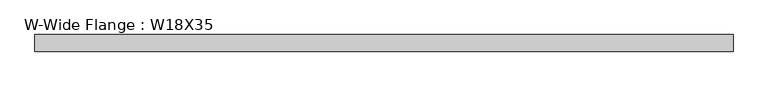
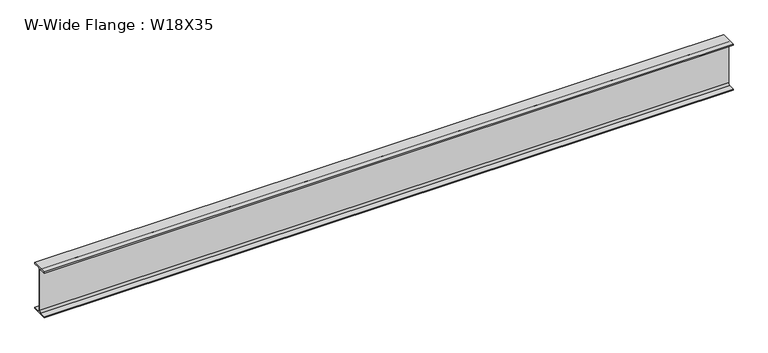
"""IFC4 building model written with IfcOpenShell, lengths in millimetres: beam geometry, W-Wide Flange : W18X35."""

from ifc_helpers import new_model, si_unit, point, frame, frame_2d, origin, place, context, project, spatial, polyline, circle_curve, trimmed, segment, composite_curve, outline, extrude, source, transform, mapped, element, save


def w_wide_flange_w18x35_87d37092(model_context):
    return source(origin(), model_context, "Body", "SweptSolid", [
        extrude(outline(composite_curve([segment(polyline([(-76.2, -213.995), (-21.59, -213.995)]), True, "CONTINUOUS"), segment(trimmed(circle_curve(frame_2d((-21.59, -196.215)), 17.78), [point((-21.59, -213.995))], [point((-3.81, -196.215))], True, "CARTESIAN"), True, "CONTINUOUS"), segment(polyline([(-3.81, -196.215), (-3.81, 196.215)]), True, "CONTINUOUS"), segment(trimmed(circle_curve(frame_2d((-21.59, 196.215)), 17.78), [point((-3.81, 196.215))], [point((-21.59, 213.995))], True, "CARTESIAN"), True, "CONTINUOUS"), segment(polyline([(-21.59, 213.995), (-76.2, 213.995), (-76.2, 224.79), (76.2, 224.79), (76.2, 213.995), (21.59, 213.995)]), True, "CONTINUOUS"), segment(trimmed(circle_curve(frame_2d((21.59, 196.215)), 17.78), [point((21.59, 213.995))], [point((3.81, 196.215))], True, "CARTESIAN"), True, "CONTINUOUS"), segment(polyline([(3.81, 196.215), (3.81, -196.215)]), True, "CONTINUOUS"), segment(trimmed(circle_curve(frame_2d((21.59, -196.215)), 17.78), [point((3.81, -196.215))], [point((21.59, -213.995))], True, "CARTESIAN"), True, "CONTINUOUS"), segment(polyline([(21.59, -213.995), (76.2, -213.995), (76.2, -224.79), (-76.2, -224.79), (-76.2, -213.995)]), True, "CONTINUOUS")], self_intersect=False)), frame((-3213.1, 0.0, 0.0), z_axis=(1.0, 0.0, 0.0), x_axis=(0.0, 1.0, 0.0)), (0.0, 0.0, 1.0), 6386.83),
    ])


if __name__ == "__main__":
    model = new_model("IFC4")
    model_context = context("Model", 3, world=origin())
    ifc_project = project(units=[si_unit("LENGTHUNIT", "METRE", prefix="MILLI")], contexts=[model_context])
    site = spatial("IfcSite", under=ifc_project)
    building = spatial("IfcBuilding", under=site)
    placement = place(None, origin())
    w_wide_flange_w18x35_shape = w_wide_flange_w18x35_87d37092(model_context)
    element("IfcBeam", 1, ObjectType="W-Wide Flange : W18X35", at=placement, inside=building, context=model_context, shape_type="MappedRepresentation", body=[
        mapped(w_wide_flange_w18x35_shape, transform((0.0, 0.0, 0.0), x_axis=(1.0, 0.0, 0.0), y_axis=(0.0, 1.0, 0.0), z_axis=(0.0, 0.0, 1.0))),
    ])
    save(model, "model.ifc")

# Revit data of these elements
# Type "W-Wide Flange : W18X35"
#   Assembly Code = "B10"
#   W = 35
#   Start Extension Calculation [instance default] = 10' - 0"
#   Start Extension [instance default] = -0' - 0 1/2"
#   End Extension Calculation [instance default] = 10' - 0"
#   End Extension [instance default] = -0' - 0 1/2"
#   Length [instance default] = 5' - 0"
#   bf = 0' - 6"
#   d = 1' - 5.7"
#   k = 0' - 1 1/8"
#   k2 = 0' - 0.7"
#   tf = 0' - 0.425"
#   tw = 0' - 0.3"
#   A = 0.0715278 SF
#   Beam Material [instance default] = Metal - Steel - ASTM A992
# Element 1 (IfcBeam, "W-Wide Flange : W18X35")
#   Materials on its faces: "Metal - Steel - ASTM A992"
# Materials
#   "Metal - Steel - ASTM A992": class "Metal", colour RGB 128 0 0, transparency 0
